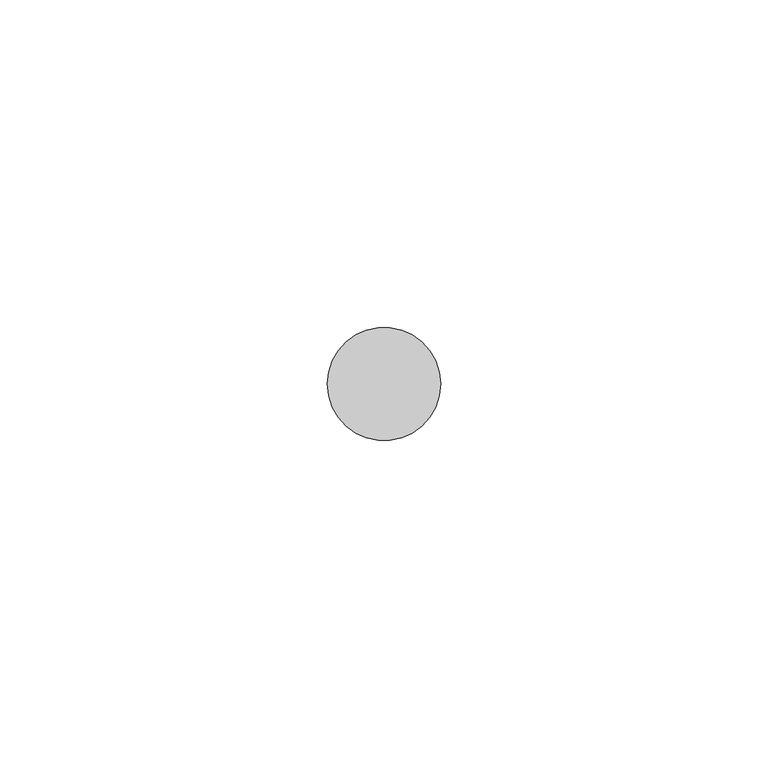
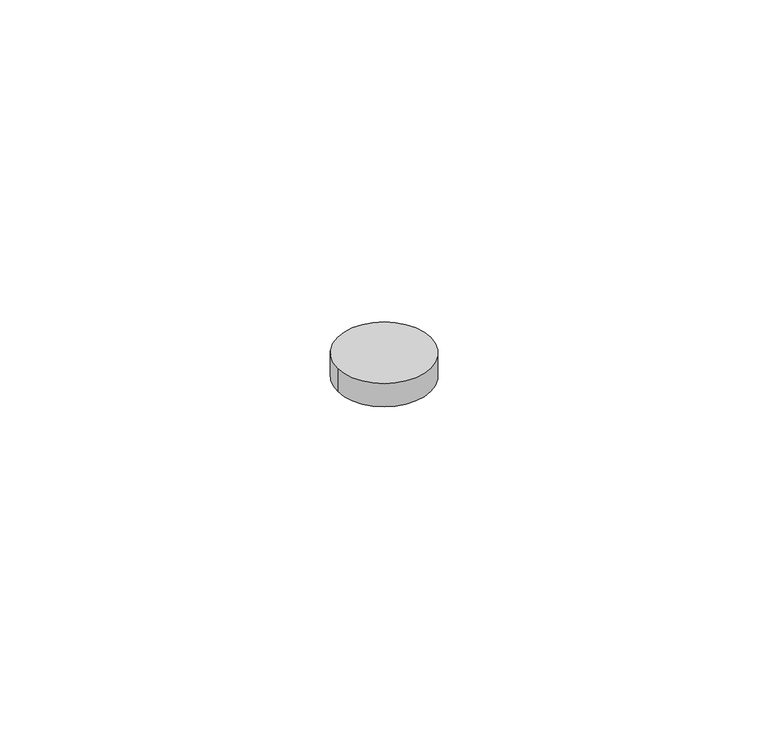
"""IFC4 building model written with IfcOpenShell, lengths in millimetres: proxy geometry, Hinge Pin Keeper3 : Hinge Pin Keeper."""

from ifc_helpers import new_model, si_unit, point, frame, frame_2d, origin, place, context, project, spatial, circle_curve, trimmed, segment, composite_curve, outline, extrude, source, transform, mapped, element, save


def generic_models_3964e635(model_context):
    return source(origin(), model_context, "Body", "SweptSolid", [
        extrude(outline(composite_curve([segment(trimmed(circle_curve(frame_2d((587319.1320739, -533984.6777841)), 8.6534625), [point((587310.4786114, -533984.6777841))], [point((587327.7855364, -533984.6777841))], False, "CARTESIAN"), True, "CONTINUOUS"), segment(trimmed(circle_curve(frame_2d((587319.1320739, -533984.6777841)), 8.6534625), [point((587327.7855364, -533984.6777841))], [point((587310.4786114, -533984.6777841))], False, "CARTESIAN"), True, "CONTINUOUS")], self_intersect=False)), frame((0.0, 0.0, 2084.5859375), z_axis=(0.0, 0.0, 1.0), x_axis=(1.0, 0.0, 0.0)), (0.0, 0.0, 1.0), 4.5640625),
    ])


if __name__ == "__main__":
    model = new_model("IFC4")
    model_context = context("Model", 3, world=origin())
    ifc_project = project(units=[si_unit("LENGTHUNIT", "METRE", prefix="MILLI")], contexts=[model_context])
    site = spatial("IfcSite", under=ifc_project)
    building = spatial("IfcBuilding", under=site)
    placement = place(None, origin())
    generic_models_shape = generic_models_3964e635(model_context)
    element("IfcBuildingElementProxy", 1, Name="Hinge Pin Keeper3 : Hinge Pin Keeper", ObjectType="Hinge Pin Keeper3 : Hinge Pin Keeper", at=placement, inside=building, context=model_context, shape_type="MappedRepresentation", body=[
        mapped(generic_models_shape, transform((0.0, 0.0, 0.0), x_axis=(1.0, 0.0, 0.0), y_axis=(0.0, 1.0, 0.0), z_axis=(0.0, 0.0, 1.0))),
    ])
    save(model, "model.ifc")

# Revit data of these elements
# Element 1 (IfcBuildingElementProxy, "Hinge Pin Keeper3 : Hinge Pin Keeper")
#   Materials on its faces: "6\"X6\" WELD-ON STL BUTT HINGE"
# Materials
#   "6\"X6\" WELD-ON STL BUTT HINGE": class "Metal", colour RGB 189 187 185, transparency 0, Description = "Carbon steel", Cost = 0
